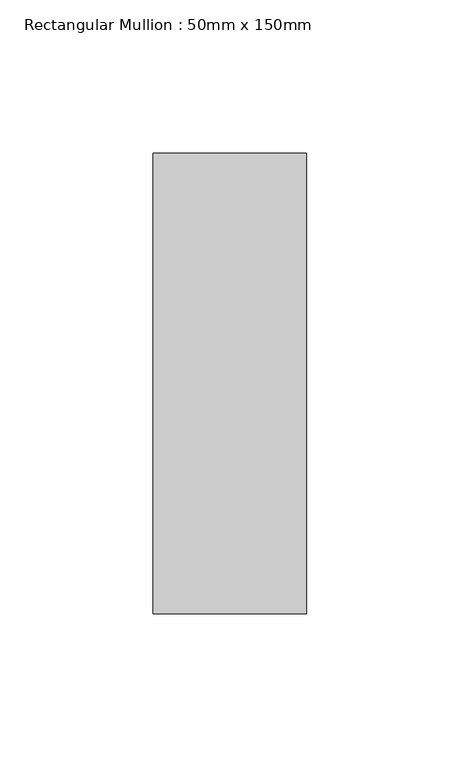
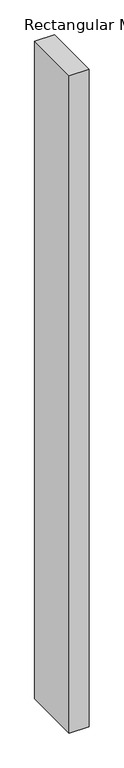
"""IFC4 building model written with IfcOpenShell, lengths in millimetres: member geometry, Rectangular Mullion : 50mm x 150mm."""

from ifc_helpers import new_model, si_unit, frame, origin, place, context, project, spatial, polyline, outline, extrude, source, transform, mapped, element, save


def rectangular_mullion_50mm_x_150mm_440fc739(model_context):
    return source(origin(), model_context, "Body", "SweptSolid", [
        extrude(outline(polyline([(0.0, 75.0), (0.0, -75.0), (-50.0, -75.0), (-50.0, 75.0), (0.0, 75.0)])), frame((0.0, 0.0, -1748.3122923), z_axis=(0.0, 0.0, 1.0), x_axis=(1.0, 0.0, 0.0)), (0.0, 0.0, 1.0), 1748.3122923),
    ])


if __name__ == "__main__":
    model = new_model("IFC4")
    model_context = context("Model", 3, world=origin())
    ifc_project = project(units=[si_unit("LENGTHUNIT", "METRE", prefix="MILLI")], contexts=[model_context])
    site = spatial("IfcSite", under=ifc_project)
    building = spatial("IfcBuilding", under=site)
    placement = place(None, origin())
    rectangular_mullion_50mm_x_150mm_shape = rectangular_mullion_50mm_x_150mm_440fc739(model_context)
    element("IfcMember", 1, ObjectType="Rectangular Mullion : 50mm x 150mm", at=placement, inside=building, context=model_context, shape_type="MappedRepresentation", body=[
        mapped(rectangular_mullion_50mm_x_150mm_shape, transform((0.0, 0.0, 0.0), x_axis=(1.0, 0.0, 0.0), y_axis=(0.0, 1.0, 0.0), z_axis=(0.0, 0.0, 1.0))),
    ])
    save(model, "model.ifc")

# Revit data of these elements
# Type "Rectangular Mullion : 50mm x 150mm"
#   built-in parameter 1007304 = 0.492126 (stored number, unit not read)
#   built-in parameter 1007301 = 0.082021 (stored number, unit not read)
#   built-in parameter 1007300 = 0.082021 (stored number, unit not read)
# Element 1 (IfcMember, "Rectangular Mullion : 50mm x 150mm")
#   Materials on its faces: "Aluminum"
# Materials
#   "Aluminum": class "Metal", colour RGB 244 244 244, transparency 0, Description = "Aluminum 6061", Cost = 0
